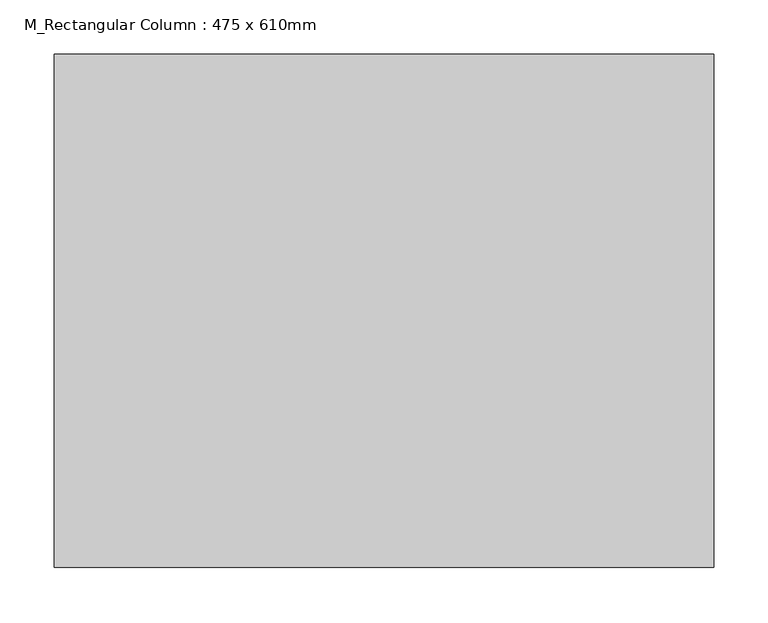
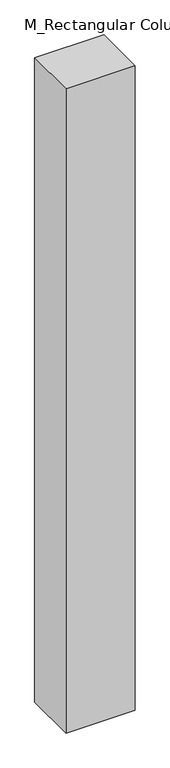
"""IFC4 building model written with IfcOpenShell, lengths in millimetres: column geometry, M_Rectangular Column : 475 x 610mm."""

from ifc_helpers import new_model, si_unit, frame, origin, place, context, project, spatial, polyline, outline, extrude, source, transform, mapped, element, save


def m_rectangular_column_475_x_610mm_a7c237de(model_context):
    return source(origin(), model_context, "Body", "SweptSolid", [
        extrude(outline(polyline([(305.0, 237.5), (305.0, -237.5), (-305.0, -237.5), (-305.0, 237.5), (305.0, 237.5)])), frame((0.0, 0.0, -2000.0), z_axis=(0.0, 0.0, 1.0), x_axis=(1.0, 0.0, 0.0)), (0.0, 0.0, 1.0), 6000.0),
    ])


if __name__ == "__main__":
    model = new_model("IFC4")
    model_context = context("Model", 3, world=origin())
    ifc_project = project(units=[si_unit("LENGTHUNIT", "METRE", prefix="MILLI")], contexts=[model_context])
    site = spatial("IfcSite", under=ifc_project)
    building = spatial("IfcBuilding", under=site)
    placement = place(None, origin())
    m_rectangular_column_475_x_610mm_shape = m_rectangular_column_475_x_610mm_a7c237de(model_context)
    element("IfcColumn", 1, ObjectType="M_Rectangular Column : 475 x 610mm", at=placement, inside=building, context=model_context, shape_type="MappedRepresentation", body=[
        mapped(m_rectangular_column_475_x_610mm_shape, transform((0.0, 0.0, 0.0), x_axis=(1.0, 0.0, 0.0), y_axis=(0.0, 1.0, 0.0), z_axis=(0.0, 0.0, 1.0))),
    ])
    save(model, "model.ifc")

# Revit data of these elements
# Type "M_Rectangular Column : 475 x 610mm"
#   Depth = 475 mm
#   Offset Base = 0 mm
#   Offset Top = 0 mm
#   Width = 610 mm
#   Material = Copper
# Element 1 (IfcColumn, "M_Rectangular Column : 475 x 610mm")
#   Materials on its faces: "Copper"
# Materials
#   "Copper": class "Metal", colour RGB 0 0 0, transparency 0, Description = "Copper, matte finish", Cost = 0
